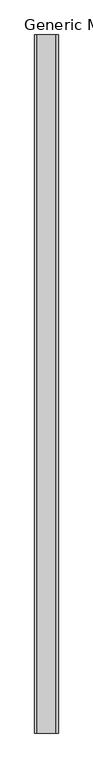
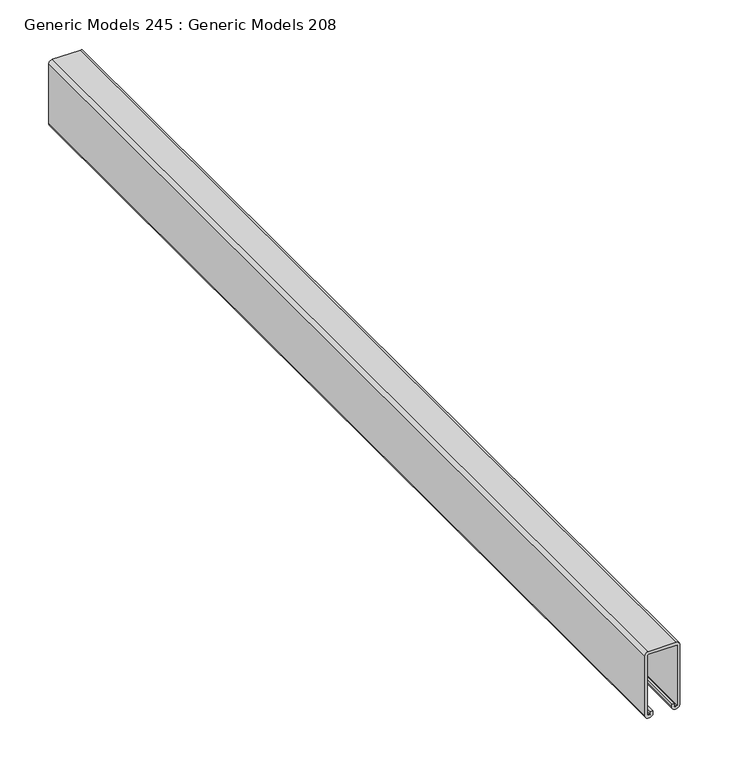
"""IFC4 building model written with IfcOpenShell, lengths in millimetres: proxy geometry, Generic Models 245 : Generic Models 208."""

from ifc_helpers import new_model, si_unit, point, frame, frame_2d, origin, place, context, project, spatial, polyline, circle_curve, trimmed, segment, composite_curve, outline, extrude, source, transform, mapped, element, save


def generic_models_245_generic_models_208_e68db20b(model_context):
    return source(origin(), model_context, "Body", "SweptSolid", [
        extrude(outline(composite_curve([segment(polyline([(2110.1689118, 53718.8649408), (2113.359375, 53718.8649408), (2113.359375, 53715.6899408), (2110.1689118, 53715.6899408)]), True, "CONTINUOUS"), segment(trimmed(circle_curve(frame_2d((2110.1689118, 53714.9116541)), 0.7782868), [point((2110.1689118, 53715.6899408))], [point((2109.390625, 53714.9116541))], True, "CARTESIAN"), True, "CONTINUOUS"), segment(polyline([(2109.390625, 53714.9116541), (2109.390625, 53713.3653996)]), True, "CONTINUOUS"), segment(trimmed(circle_curve(frame_2d((2110.2410838, 53713.3653996)), 0.8504588), [point((2109.390625, 53713.3653996))], [point((2110.2410838, 53712.5149408))], True, "CARTESIAN"), True, "CONTINUOUS"), segment(polyline([(2110.2410838, 53712.5149408), (2184.7417804, 53712.5149408)]), True, "CONTINUOUS"), segment(trimmed(circle_curve(frame_2d((2184.7417804, 53713.3637855)), 0.8488446), [point((2184.7417804, 53712.5149408))], [point((2185.590625, 53713.3637855))], True, "CARTESIAN"), True, "CONTINUOUS"), segment(polyline([(2185.590625, 53713.3637855), (2185.590625, 53746.6306179)]), True, "CONTINUOUS"), segment(trimmed(circle_curve(frame_2d((2184.7813021, 53746.6306179)), 0.8093229), [point((2185.590625, 53746.6306179))], [point((2184.7813021, 53747.4399408))], True, "CARTESIAN"), True, "CONTINUOUS"), segment(polyline([(2184.7813021, 53747.4399408), (2110.2275339, 53747.4399408)]), True, "CONTINUOUS"), segment(trimmed(circle_curve(frame_2d((2110.2275339, 53746.6030319)), 0.8369089), [point((2110.2275339, 53747.4399408))], [point((2109.390625, 53746.6030319))], True, "CARTESIAN"), True, "CONTINUOUS"), segment(polyline([(2109.390625, 53746.6030319), (2109.390625, 53745.1342437)]), True, "CONTINUOUS"), segment(trimmed(circle_curve(frame_2d((2110.2599279, 53745.1342437)), 0.8693029), [point((2109.390625, 53745.1342437))], [point((2110.2599279, 53744.2649408))], True, "CARTESIAN"), True, "CONTINUOUS"), segment(polyline([(2110.2599279, 53744.2649408), (2113.359375, 53744.2649408), (2113.359375, 53741.0899408), (2110.2599279, 53741.0899408)]), True, "CONTINUOUS"), segment(trimmed(circle_curve(frame_2d((2110.2599279, 53745.1342437)), 4.0443029), [point((2110.2599279, 53741.0899408))], [point((2106.215625, 53745.1342437))], False, "CARTESIAN"), True, "CONTINUOUS"), segment(polyline([(2106.215625, 53745.1342437), (2106.215625, 53746.6030319)]), True, "CONTINUOUS"), segment(trimmed(circle_curve(frame_2d((2110.2275339, 53746.6030319)), 4.0119089), [point((2106.215625, 53746.6030319))], [point((2110.2275339, 53750.6149408))], False, "CARTESIAN"), True, "CONTINUOUS"), segment(polyline([(2110.2275339, 53750.6149408), (2184.7813021, 53750.6149408)]), True, "CONTINUOUS"), segment(trimmed(circle_curve(frame_2d((2184.7813021, 53746.6306179)), 3.9843229), [point((2184.7813021, 53750.6149408))], [point((2188.765625, 53746.6306179))], False, "CARTESIAN"), True, "CONTINUOUS"), segment(polyline([(2188.765625, 53746.6306179), (2188.765625, 53713.3637855)]), True, "CONTINUOUS"), segment(trimmed(circle_curve(frame_2d((2184.7417804, 53713.3637855)), 4.0238446), [point((2188.765625, 53713.3637855))], [point((2184.7417804, 53709.3399408))], False, "CARTESIAN"), True, "CONTINUOUS"), segment(polyline([(2184.7417804, 53709.3399408), (2110.2410838, 53709.3399408)]), True, "CONTINUOUS"), segment(trimmed(circle_curve(frame_2d((2110.2410838, 53713.3653996)), 4.0254588), [point((2110.2410838, 53709.3399408))], [point((2106.215625, 53713.3653996))], False, "CARTESIAN"), True, "CONTINUOUS"), segment(polyline([(2106.215625, 53713.3653996), (2106.215625, 53714.9116541)]), True, "CONTINUOUS"), segment(trimmed(circle_curve(frame_2d((2110.1689118, 53714.9116541)), 3.9532868), [point((2106.215625, 53714.9116541))], [point((2110.1689118, 53718.8649408))], False, "CARTESIAN"), True, "CONTINUOUS")], self_intersect=False)), frame((0.0, -228.7033818, 0.0), z_axis=(0.0, 1.0, 0.0), x_axis=(0.0, 0.0, 1.0)), (0.0, 0.0, 1.0), 1219.2),
    ])


if __name__ == "__main__":
    model = new_model("IFC4")
    model_context = context("Model", 3, world=origin())
    ifc_project = project(units=[si_unit("LENGTHUNIT", "METRE", prefix="MILLI")], contexts=[model_context])
    site = spatial("IfcSite", under=ifc_project)
    building = spatial("IfcBuilding", under=site)
    placement = place(None, origin())
    generic_models_245_generic_models_208_shape = generic_models_245_generic_models_208_e68db20b(model_context)
    element("IfcBuildingElementProxy", 1, Name="Generic Models 245 : Generic Models 208", ObjectType="Generic Models 245 : Generic Models 208", at=placement, inside=building, context=model_context, shape_type="MappedRepresentation", body=[
        mapped(generic_models_245_generic_models_208_shape, transform((0.0, 0.0, 0.0), x_axis=(1.0, 0.0, 0.0), y_axis=(0.0, 1.0, 0.0), z_axis=(0.0, 0.0, 1.0))),
    ])
    save(model, "model.ifc")

# Revit data of these elements
# Element 1 (IfcBuildingElementProxy, "Generic Models 245 : Generic Models 208")
#   Materials on its faces: "UNISTRUT P5000, 1-5/8\" x 3-1/4\", 12 GA METAL FRAMING CHANNEL STRUT"
# Materials
#   "UNISTRUT P5000, 1-5/8\" x 3-1/4\", 12 GA METAL FRAMING CHANNEL STRUT": class "Metal", colour RGB 244 244 244, transparency 0, Description = "Aluminum 6061", Cost = 0
